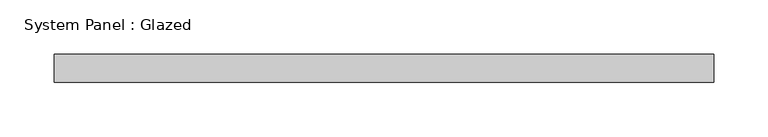
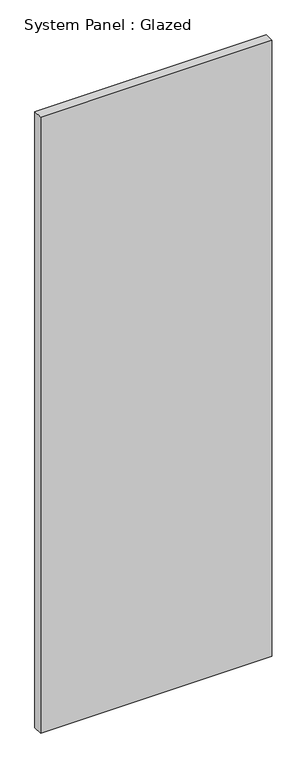
"""IFC4 building model written with IfcOpenShell, lengths in millimetres: plate geometry, System Panel : Glazed."""

from ifc_helpers import new_model, si_unit, origin, origin_with_axes, place, context, project, spatial, polyline, outline, extrude, source, transform, mapped, element, save


def system_panel_glazed_35f19b2b(model_context):
    return source(origin(), model_context, "Body", "SweptSolid", [
        extrude(outline(polyline([(302.375, 19.05), (-302.375, 19.05), (-302.375, 44.45), (302.375, 44.45), (302.375, 19.05)])), origin_with_axes(), (0.0, 0.0, 1.0), 1701.8),
    ])


if __name__ == "__main__":
    model = new_model("IFC4")
    model_context = context("Model", 3, world=origin())
    ifc_project = project(units=[si_unit("LENGTHUNIT", "METRE", prefix="MILLI")], contexts=[model_context])
    site = spatial("IfcSite", under=ifc_project)
    building = spatial("IfcBuilding", under=site)
    placement = place(None, origin())
    system_panel_glazed_shape = system_panel_glazed_35f19b2b(model_context)
    element("IfcPlate", 1, ObjectType="System Panel : Glazed", at=placement, inside=building, context=model_context, shape_type="MappedRepresentation", body=[
        mapped(system_panel_glazed_shape, transform((0.0, 0.0, 0.0), x_axis=(1.0, 0.0, 0.0), y_axis=(0.0, 1.0, 0.0), z_axis=(0.0, 0.0, 1.0))),
    ])
    save(model, "model.ifc")

# Revit data of these elements
# Element 1 (IfcPlate, "System Panel : Glazed")
#   Materials on its faces: "Glass"
# Materials
#   "Glass": class "Glass", colour RGB 0 128 192, transparency 0.75
